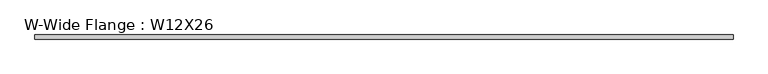
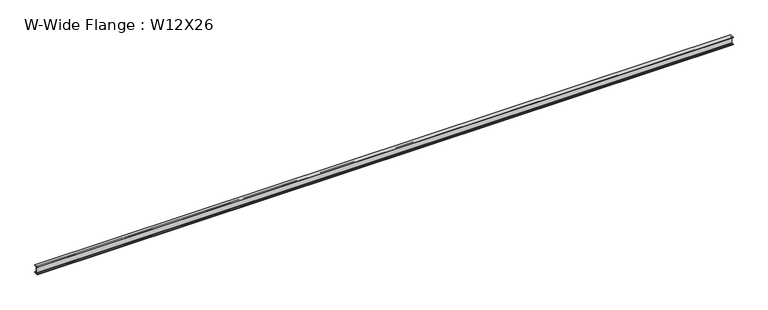
"""IFC4 building model written with IfcOpenShell, lengths in millimetres: beam geometry, W-Wide Flange : W12X26."""

from ifc_helpers import new_model, si_unit, point, frame, frame_2d, origin, place, context, project, spatial, polyline, circle_curve, trimmed, segment, composite_curve, outline, extrude, source, transform, mapped, element, save


def w_wide_flange_w12x26_0a813f0e(model_context):
    return source(origin(), model_context, "Body", "SweptSolid", [
        extrude(outline(composite_curve([segment(polyline([(82.4011719, -145.5539063), (82.4011719, -155.178125), (-82.4011719, -155.178125), (-82.4011719, -145.5539063), (-20.2902344, -145.5539063)]), True, "CONTINUOUS"), segment(trimmed(circle_curve(frame_2d((-20.2902344, -128.190625)), 17.3632812), [point((-20.2902344, -145.5539063))], [point((-2.9269531, -128.190625))], True, "CARTESIAN"), True, "CONTINUOUS"), segment(polyline([(-2.9269531, -128.190625), (-2.9269531, 128.190625)]), True, "CONTINUOUS"), segment(trimmed(circle_curve(frame_2d((-20.2902344, 128.190625)), 17.3632812), [point((-2.9269531, 128.190625))], [point((-20.2902344, 145.5539062))], True, "CARTESIAN"), True, "CONTINUOUS"), segment(polyline([(-20.2902344, 145.5539062), (-82.4011719, 145.5539062), (-82.4011719, 155.178125), (82.4011719, 155.178125), (82.4011719, 145.5539062), (20.2902344, 145.5539062)]), True, "CONTINUOUS"), segment(trimmed(circle_curve(frame_2d((20.2902344, 128.190625)), 17.3632812), [point((20.2902344, 145.5539062))], [point((2.9269531, 128.190625))], True, "CARTESIAN"), True, "CONTINUOUS"), segment(polyline([(2.9269531, 128.190625), (2.9269531, -128.190625)]), True, "CONTINUOUS"), segment(trimmed(circle_curve(frame_2d((20.2902344, -128.190625)), 17.3632812), [point((2.9269531, -128.190625))], [point((20.2902344, -145.5539063))], True, "CARTESIAN"), True, "CONTINUOUS"), segment(polyline([(20.2902344, -145.5539063), (82.4011719, -145.5539063)]), True, "CONTINUOUS")], self_intersect=False)), frame((-25624.0113662, 0.0, 0.0), z_axis=(1.0, 0.0, 0.0), x_axis=(0.0, 1.0, 0.0)), (0.0, 0.0, 1.0), 27573.8603238),
    ])


if __name__ == "__main__":
    model = new_model("IFC4")
    model_context = context("Model", 3, world=origin())
    ifc_project = project(units=[si_unit("LENGTHUNIT", "METRE", prefix="MILLI")], contexts=[model_context])
    site = spatial("IfcSite", under=ifc_project)
    building = spatial("IfcBuilding", under=site)
    placement = place(None, origin())
    w_wide_flange_w12x26_shape = w_wide_flange_w12x26_0a813f0e(model_context)
    element("IfcBeam", 1, ObjectType="W-Wide Flange : W12X26", at=placement, inside=building, context=model_context, shape_type="MappedRepresentation", body=[
        mapped(w_wide_flange_w12x26_shape, transform((0.0, 0.0, 0.0), x_axis=(1.0, 0.0, 0.0), y_axis=(0.0, 1.0, 0.0), z_axis=(0.0, 0.0, 1.0))),
    ])
    save(model, "model.ifc")

# Revit data of these elements
# Type "W-Wide Flange : W12X26"
#   Assembly Code = "B10"
#   W = 26
#   Length [instance default] = 5' - 0"
#   bf = 0' - 6 125/256"
#   d = 1' - 0 7/32"
#   k = 0' - 1 1/16"
#   k2 = 0' - 0 175/256"
#   tf = 0' - 0 97/256"
#   tw = 0' - 0 59/256"
#   A = 0.053125 SF
#   Structural Material [instance default] = none
